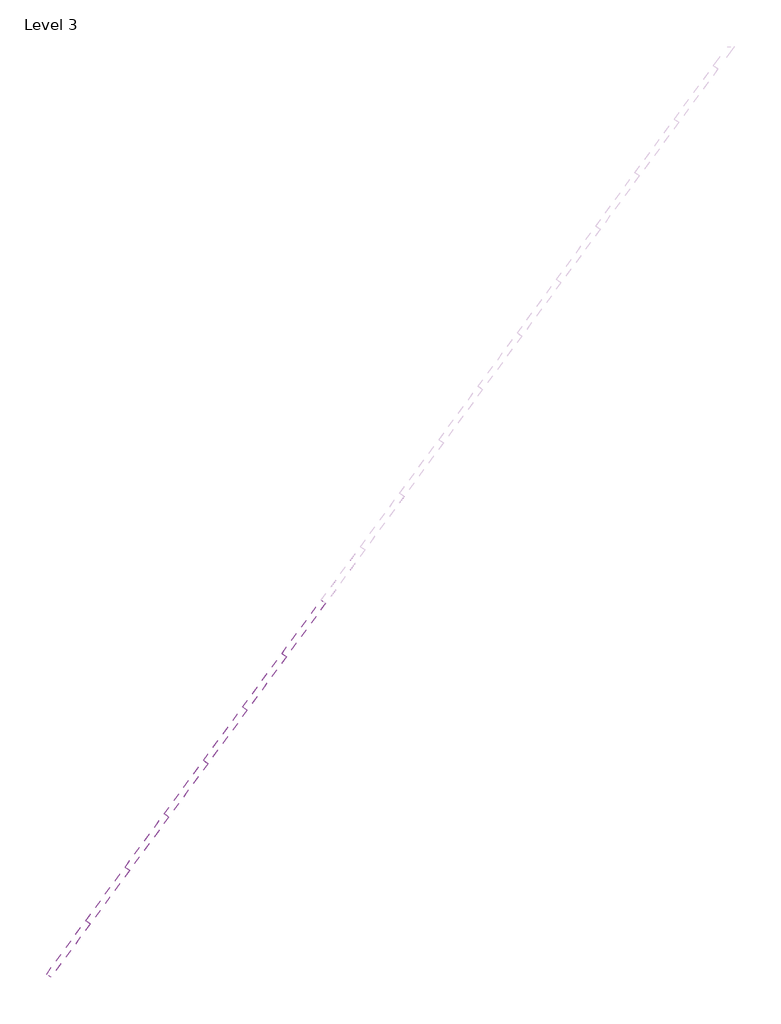
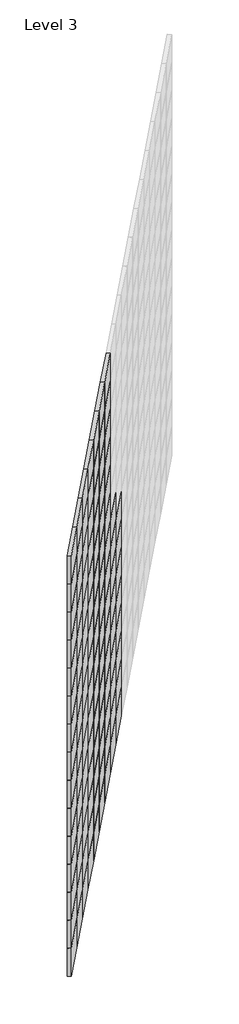
# One storey, part 1 of 9: 122 plates.
"""IFC4 building model written with IfcOpenShell, lengths in millimetres."""

import ifcopenshell
import ifcopenshell.guid

model = None  # the IFC model being written
_history = None  # IfcOwnerHistory: only IFC2X3 demands one
_inside = {}  # id of a spatial element -> (the spatial element, [elements in it])
_under = {}  # id of a project, library or spatial element -> (it, [spatial elements below it])
_declared = {}  # id of a project -> (the project, [libraries it declares])
_typed = {}  # id of a type object -> (the type object, [elements of that type])
_made_of = {}  # id of a material, layer set ... -> (it, [elements and type objects made of it])


def new_model(schema):
    """Start an empty IFC model of exactly this schema.

    Asked for "IFC4X3", IfcOpenShell would pick the latest addendum, in which some entities
    have other attributes; the version numbers below select the first issue.
    IFC2X3 requires an IfcOwnerHistory on every rooted entity: one is made here for all.
    """
    global model, _history
    if schema == "IFC4X3":
        model = ifcopenshell.file(schema_version=(4, 3, 0, 0))
    else:
        model = ifcopenshell.file(schema=schema)
    _inside.clear()
    _under.clear()
    _declared.clear()
    _typed.clear()
    _made_of.clear()
    _history = None
    if model.schema == "IFC2X3":
        org = make("IfcOrganization", Name="unknown")
        user = make(
            "IfcPersonAndOrganization",
            ThePerson=make("IfcPerson", FamilyName="unknown"),
            TheOrganization=org,
        )
        app = make(
            "IfcApplication",
            ApplicationDeveloper=org,
            Version="unknown",
            ApplicationFullName="unknown",
            ApplicationIdentifier="unknown",
        )
        _history = make(
            "IfcOwnerHistory",
            OwningUser=user,
            OwningApplication=app,
            ChangeAction="ADDED",
            CreationDate=0,
        )
    return model


def make(cls, **values):
    """One entity of the class cls with the attributes given. An attribute that is None is left unset."""
    return model.create_entity(
        cls, **{name: value for name, value in values.items() if value is not None}
    )


def rooted(cls, **values):
    """An entity with a GlobalId (a new one), such as an element, a storey or a relation."""
    return make(cls, GlobalId=ifcopenshell.guid.new(), OwnerHistory=_history, **values)


def si_unit(unit_type, name, prefix=None):
    """IfcSIUnit, for example si_unit("LENGTHUNIT", "METRE", prefix="MILLI")."""
    return make("IfcSIUnit", UnitType=unit_type, Prefix=prefix, Name=name)


def assignment(units):
    """IfcUnitAssignment: the units of a project."""
    return None if units is None else make("IfcUnitAssignment", Units=units)


def point(xyz):
    """IfcCartesianPoint."""
    return None if xyz is None else make("IfcCartesianPoint", Coordinates=xyz)


def direction(xyz):
    """IfcDirection."""
    return None if xyz is None else make("IfcDirection", DirectionRatios=xyz)


def frame(location, z_axis=None, x_axis=None):
    """IfcAxis2Placement3D, a coordinate frame: its origin and axes. An axis left out is left unset."""
    return make(
        "IfcAxis2Placement3D",
        Location=point(location),
        Axis=direction(z_axis),
        RefDirection=direction(x_axis),
    )


def origin():
    """The frame at (0, 0, 0) with its axes left unset."""
    return frame((0.0, 0.0, 0.0))


def origin_with_axes():
    """The frame at (0, 0, 0) with the z axis (0, 0, 1) and the x axis (1, 0, 0) written out."""
    return frame((0.0, 0.0, 0.0), z_axis=(0.0, 0.0, 1.0), x_axis=(1.0, 0.0, 0.0))


def place(relative_to, where):
    """IfcLocalPlacement: puts the frame where relative to a parent placement (None: the world)."""
    return make(
        "IfcLocalPlacement", PlacementRelTo=relative_to, RelativePlacement=where
    )


def context(
    kind, dimensions, precision=None, world=None, true_north=None, identifier=None
):
    """IfcGeometricRepresentationContext, for example the 3D "Model" context."""
    return make(
        "IfcGeometricRepresentationContext",
        ContextIdentifier=identifier,
        ContextType=kind,
        CoordinateSpaceDimension=dimensions,
        Precision=precision,
        WorldCoordinateSystem=world,
        TrueNorth=true_north,
    )


def project(units=None, contexts=None):
    """IfcProject with its units and contexts."""
    return rooted(
        "IfcProject",
        Name="project",
        RepresentationContexts=contexts,
        UnitsInContext=assignment(units),
    )


def spatial(cls, under=None, at=None, **own):
    """A site, building, storey or space (cls), placed at a placement, below another one or the project."""
    s = rooted(cls, ObjectPlacement=at, **own)
    if under is not None:
        _under.setdefault(under.id(), (under, []))[1].append(s)
    return s


def polyline(points):
    """IfcPolyline through the points."""
    return make("IfcPolyline", Points=[point(p) for p in points])


def outline(outer, holes=None, kind="AREA"):
    """IfcArbitraryClosedProfileDef: a profile drawn as a closed curve; with holes, ...WithVoids."""
    if holes is None:
        return make("IfcArbitraryClosedProfileDef", ProfileType=kind, OuterCurve=outer)
    return make(
        "IfcArbitraryProfileDefWithVoids",
        ProfileType=kind,
        OuterCurve=outer,
        InnerCurves=holes,
    )


def extrude(swept, where, along, depth):
    """IfcExtrudedAreaSolid: the profile swept, set in the frame where, extruded along a direction by depth."""
    return make(
        "IfcExtrudedAreaSolid",
        SweptArea=swept,
        Position=where,
        ExtrudedDirection=direction(along),
        Depth=depth,
    )


def shape(context_of_items, identifier, shape_type, items):
    """IfcShapeRepresentation: the items that make up one representation, for example the "Body"."""
    return make(
        "IfcShapeRepresentation",
        ContextOfItems=context_of_items,
        RepresentationIdentifier=identifier,
        RepresentationType=shape_type,
        Items=items,
    )


def source(mapping_origin, context_of_items, identifier, shape_type, items):
    """IfcRepresentationMap: a shape defined once, which mapped items show again and again."""
    return make(
        "IfcRepresentationMap",
        MappingOrigin=mapping_origin,
        MappedRepresentation=shape(context_of_items, identifier, shape_type, items),
    )


def transform(
    local_origin,
    x_axis=None,
    y_axis=None,
    z_axis=None,
    scale=None,
    scale2=None,
    scale3=None,
    uniform=True,
):
    """IfcCartesianTransformationOperator3D, or its non-uniform kind. x_axis, y_axis, z_axis: its Axis1, 2, 3."""
    if uniform:
        return make(
            "IfcCartesianTransformationOperator3D",
            Axis1=direction(x_axis),
            Axis2=direction(y_axis),
            LocalOrigin=point(local_origin),
            Scale=scale,
            Axis3=direction(z_axis),
        )
    return make(
        "IfcCartesianTransformationOperator3DnonUniform",
        Axis1=direction(x_axis),
        Axis2=direction(y_axis),
        LocalOrigin=point(local_origin),
        Scale=scale,
        Axis3=direction(z_axis),
        Scale2=scale2,
        Scale3=scale3,
    )


def mapped(mapping_source, mapping_target):
    """IfcMappedItem: shows the shape of a source again, moved by a transform."""
    return make(
        "IfcMappedItem", MappingSource=mapping_source, MappingTarget=mapping_target
    )


def made_of(thing, what):
    """Note that an element or type object is made of a material, layer set ...; save() writes the relation."""
    if what is not None:
        _made_of.setdefault(what.id(), (what, []))[1].append(thing)
    return thing


def element(
    cls,
    number,
    at=None,
    inside=None,
    cuts=None,
    type_object=None,
    material=None,
    context=None,
    identifier="Body",
    shape_type=None,
    held_by="IfcProductDefinitionShape",
    body=None,
    shapes=None,
    **own,
):
    """One element of the class cls, such as IfcWall. Its Tag is "e" and its number.

    at: its placement. inside: the storey or other place that contains it. cuts: it is an
    opening in that element (IfcRelVoidsElement). A single representation is given by context,
    identifier, shape_type and body (its items); several are given by shapes. held_by: the class
    of the entity that holds the representations. save() writes the other relations.
    """
    e = rooted(cls, Tag="e%d" % number, ObjectPlacement=at, **own)
    if body is not None:
        shapes = [shape(context, identifier, shape_type, body)]
    if shapes is not None:
        e.Representation = make(held_by, Representations=shapes)
    if inside is not None:
        _inside.setdefault(inside.id(), (inside, []))[1].append(e)
    if cuts is not None:
        rooted(
            "IfcRelVoidsElement", RelatingBuildingElement=cuts, RelatedOpeningElement=e
        )
    if type_object is not None:
        _typed.setdefault(type_object.id(), (type_object, []))[1].append(e)
    return made_of(e, material)


def aggregate(whole, parts):
    """IfcRelAggregates: a whole, such as a stair, and the parts it consists of."""
    return rooted("IfcRelAggregates", RelatingObject=whole, RelatedObjects=parts)


def save(model, path):
    """Write the relations noted so far, then the file.

    IfcRelAggregates (storeys below a building ...), IfcRelContainedInSpatialStructure (elements
    in a storey), IfcRelDefinesByType, IfcRelAssociatesMaterial and IfcRelDeclares: one each for
    every whole, place, type object, material and project.
    """
    for whole, parts in _under.values():
        aggregate(whole, parts)
    for where, things in _inside.values():
        rooted(
            "IfcRelContainedInSpatialStructure",
            RelatedElements=things,
            RelatingStructure=where,
        )
    for kind, things in _typed.values():
        rooted("IfcRelDefinesByType", RelatedObjects=things, RelatingType=kind)
    for what, things in _made_of.values():
        rooted("IfcRelAssociatesMaterial", RelatedObjects=things, RelatingMaterial=what)
    for by, libraries in _declared.values():
        rooted("IfcRelDeclares", RelatingContext=by, RelatedDefinitions=libraries)
    model.write(path)


def system_panel_glazed_2fc8f5ca(model_context):
    return source(origin(), model_context, "Body", "SweptSolid", [
        extrude(outline(polyline([(148.4832393, 24.5), (-148.4832393, 24.5), (-148.4832393, 49.5), (148.4832393, 49.5), (148.4832393, 24.5)])), origin_with_axes(), (0.0, 0.0, 1.0), 200.0),
    ])


model = new_model("IFC4")

# Units and contexts
model_context = context("Model", 3, world=origin())
ifc_project = project(units=[si_unit("LENGTHUNIT", "METRE", prefix="MILLI")], contexts=[model_context])

# Site, building, storey
site = spatial("IfcSite", under=ifc_project)
building = spatial("IfcBuilding", under=site)
storey = spatial("IfcBuildingStorey", under=building, Name="Level 3", Elevation=22950.0)

# Plates
placement = place(None, origin())
system_panel_glazed_shape = system_panel_glazed_2fc8f5ca(model_context)
element("IfcPlate", 1, ObjectType="System Panel : Glazed", at=placement, inside=storey, context=model_context, shape_type="MappedRepresentation", body=[
    mapped(system_panel_glazed_shape, transform((-37416.3631886, 22522.5700791, 35100.0), x_axis=(0.5920548138930122, 0.8058976965757569, 0.0), y_axis=(-0.8058976965757569, 0.5920548138930122, 0.0), z_axis=(0.0, 0.0, 1.0))),
])
element("IfcPlate", 2, ObjectType="System Panel : Glazed", at=placement, inside=storey, context=model_context, shape_type="MappedRepresentation", body=[
    mapped(system_panel_glazed_shape, transform((-37240.5427555, 22761.8946801, 35100.0), x_axis=(0.5920548138930122, 0.8058976965757569, 0.0), y_axis=(-0.8058976965757569, 0.5920548138930122, 0.0), z_axis=(0.0, 0.0, 1.0))),
])
element("IfcPlate", 3, ObjectType="System Panel : Glazed", at=placement, inside=storey, context=model_context, shape_type="MappedRepresentation", body=[
    mapped(system_panel_glazed_shape, transform((-37064.7223224, 23001.2192809, 35100.0), x_axis=(0.5920548138930122, 0.8058976965757569, 0.0), y_axis=(-0.8058976965757569, 0.5920548138930122, 0.0), z_axis=(0.0, 0.0, 1.0))),
])
element("IfcPlate", 4, ObjectType="System Panel : Glazed", at=placement, inside=storey, context=model_context, shape_type="MappedRepresentation", body=[
    mapped(system_panel_glazed_shape, transform((-36888.9018893, 23240.5438818, 35100.0), x_axis=(0.5920548138930122, 0.8058976965757569, 0.0), y_axis=(-0.8058976965757569, 0.5920548138930122, 0.0), z_axis=(0.0, 0.0, 1.0))),
])
element("IfcPlate", 5, ObjectType="System Panel : Glazed", at=placement, inside=storey, context=model_context, shape_type="MappedRepresentation", body=[
    mapped(system_panel_glazed_shape, transform((-36713.0814563, 23479.8684826, 35100.0), x_axis=(0.5920548138930122, 0.8058976965757569, 0.0), y_axis=(-0.8058976965757569, 0.5920548138930122, 0.0), z_axis=(0.0, 0.0, 1.0))),
])
element("IfcPlate", 6, ObjectType="System Panel : Glazed", at=placement, inside=storey, context=model_context, shape_type="MappedRepresentation", body=[
    mapped(system_panel_glazed_shape, transform((-36537.2610232, 23719.1930834, 35100.0), x_axis=(0.5920548138930122, 0.8058976965757569, 0.0), y_axis=(-0.8058976965757569, 0.5920548138930122, 0.0), z_axis=(0.0, 0.0, 1.0))),
])
element("IfcPlate", 7, ObjectType="System Panel : Glazed", at=placement, inside=storey, context=model_context, shape_type="MappedRepresentation", body=[
    mapped(system_panel_glazed_shape, transform((-36361.4405902, 23958.5176843, 35100.0), x_axis=(0.5920548138930122, 0.8058976965757569, 0.0), y_axis=(-0.8058976965757569, 0.5920548138930122, 0.0), z_axis=(0.0, 0.0, 1.0))),
])
element("IfcPlate", 8, ObjectType="System Panel : Glazed", at=placement, inside=storey, context=model_context, shape_type="MappedRepresentation", body=[
    mapped(system_panel_glazed_shape, transform((-36185.6201571, 24197.8422851, 35100.0), x_axis=(0.5920548138930122, 0.8058976965757569, 0.0), y_axis=(-0.8058976965757569, 0.5920548138930122, 0.0), z_axis=(0.0, 0.0, 1.0))),
])
element("IfcPlate", 9, ObjectType="System Panel : Glazed", at=placement, inside=storey, context=model_context, shape_type="MappedRepresentation", body=[
    mapped(system_panel_glazed_shape, transform((-36009.7997241, 24437.166886, 35100.0), x_axis=(0.5920548138930122, 0.8058976965757569, 0.0), y_axis=(-0.8058976965757569, 0.5920548138930122, 0.0), z_axis=(0.0, 0.0, 1.0))),
])
element("IfcPlate", 10, ObjectType="System Panel : Glazed", at=placement, inside=storey, context=model_context, shape_type="MappedRepresentation", body=[
    mapped(system_panel_glazed_shape, transform((-37416.3631886, 22522.5700791, 35300.0), x_axis=(0.5920548138930122, 0.8058976965757569, 0.0), y_axis=(-0.8058976965757569, 0.5920548138930122, 0.0), z_axis=(0.0, 0.0, 1.0))),
])
element("IfcPlate", 11, ObjectType="System Panel : Glazed", at=placement, inside=storey, context=model_context, shape_type="MappedRepresentation", body=[
    mapped(system_panel_glazed_shape, transform((-37240.5427555, 22761.8946801, 35300.0), x_axis=(0.5920548138930122, 0.8058976965757569, 0.0), y_axis=(-0.8058976965757569, 0.5920548138930122, 0.0), z_axis=(0.0, 0.0, 1.0))),
])
element("IfcPlate", 12, ObjectType="System Panel : Glazed", at=placement, inside=storey, context=model_context, shape_type="MappedRepresentation", body=[
    mapped(system_panel_glazed_shape, transform((-37064.7223224, 23001.2192809, 35300.0), x_axis=(0.5920548138930122, 0.8058976965757569, 0.0), y_axis=(-0.8058976965757569, 0.5920548138930122, 0.0), z_axis=(0.0, 0.0, 1.0))),
])
element("IfcPlate", 13, ObjectType="System Panel : Glazed", at=placement, inside=storey, context=model_context, shape_type="MappedRepresentation", body=[
    mapped(system_panel_glazed_shape, transform((-36888.9018893, 23240.5438818, 35300.0), x_axis=(0.5920548138930122, 0.8058976965757569, 0.0), y_axis=(-0.8058976965757569, 0.5920548138930122, 0.0), z_axis=(0.0, 0.0, 1.0))),
])
element("IfcPlate", 14, ObjectType="System Panel : Glazed", at=placement, inside=storey, context=model_context, shape_type="MappedRepresentation", body=[
    mapped(system_panel_glazed_shape, transform((-36713.0814563, 23479.8684826, 35300.0), x_axis=(0.5920548138930122, 0.8058976965757569, 0.0), y_axis=(-0.8058976965757569, 0.5920548138930122, 0.0), z_axis=(0.0, 0.0, 1.0))),
])
element("IfcPlate", 15, ObjectType="System Panel : Glazed", at=placement, inside=storey, context=model_context, shape_type="MappedRepresentation", body=[
    mapped(system_panel_glazed_shape, transform((-36537.2610232, 23719.1930834, 35300.0), x_axis=(0.5920548138930122, 0.8058976965757569, 0.0), y_axis=(-0.8058976965757569, 0.5920548138930122, 0.0), z_axis=(0.0, 0.0, 1.0))),
])
element("IfcPlate", 16, ObjectType="System Panel : Glazed", at=placement, inside=storey, context=model_context, shape_type="MappedRepresentation", body=[
    mapped(system_panel_glazed_shape, transform((-36361.4405902, 23958.5176843, 35300.0), x_axis=(0.5920548138930122, 0.8058976965757569, 0.0), y_axis=(-0.8058976965757569, 0.5920548138930122, 0.0), z_axis=(0.0, 0.0, 1.0))),
])
element("IfcPlate", 17, ObjectType="System Panel : Glazed", at=placement, inside=storey, context=model_context, shape_type="MappedRepresentation", body=[
    mapped(system_panel_glazed_shape, transform((-36185.6201571, 24197.8422851, 35300.0), x_axis=(0.5920548138930122, 0.8058976965757569, 0.0), y_axis=(-0.8058976965757569, 0.5920548138930122, 0.0), z_axis=(0.0, 0.0, 1.0))),
])
element("IfcPlate", 18, ObjectType="System Panel : Glazed", at=placement, inside=storey, context=model_context, shape_type="MappedRepresentation", body=[
    mapped(system_panel_glazed_shape, transform((-36009.7997241, 24437.166886, 35300.0), x_axis=(0.5920548138930122, 0.8058976965757569, 0.0), y_axis=(-0.8058976965757569, 0.5920548138930122, 0.0), z_axis=(0.0, 0.0, 1.0))),
])
element("IfcPlate", 19, ObjectType="System Panel : Glazed", at=placement, inside=storey, context=model_context, shape_type="MappedRepresentation", body=[
    mapped(system_panel_glazed_shape, transform((-37416.3631886, 22522.5700791, 35500.0), x_axis=(0.5920548138930122, 0.8058976965757569, 0.0), y_axis=(-0.8058976965757569, 0.5920548138930122, 0.0), z_axis=(0.0, 0.0, 1.0))),
])
element("IfcPlate", 20, ObjectType="System Panel : Glazed", at=placement, inside=storey, context=model_context, shape_type="MappedRepresentation", body=[
    mapped(system_panel_glazed_shape, transform((-37240.5427555, 22761.8946801, 35500.0), x_axis=(0.5920548138930122, 0.8058976965757569, 0.0), y_axis=(-0.8058976965757569, 0.5920548138930122, 0.0), z_axis=(0.0, 0.0, 1.0))),
])
element("IfcPlate", 21, ObjectType="System Panel : Glazed", at=placement, inside=storey, context=model_context, shape_type="MappedRepresentation", body=[
    mapped(system_panel_glazed_shape, transform((-37064.7223224, 23001.2192809, 35500.0), x_axis=(0.5920548138930122, 0.8058976965757569, 0.0), y_axis=(-0.8058976965757569, 0.5920548138930122, 0.0), z_axis=(0.0, 0.0, 1.0))),
])
element("IfcPlate", 22, ObjectType="System Panel : Glazed", at=placement, inside=storey, context=model_context, shape_type="MappedRepresentation", body=[
    mapped(system_panel_glazed_shape, transform((-36888.9018893, 23240.5438818, 35500.0), x_axis=(0.5920548138930122, 0.8058976965757569, 0.0), y_axis=(-0.8058976965757569, 0.5920548138930122, 0.0), z_axis=(0.0, 0.0, 1.0))),
])
element("IfcPlate", 23, ObjectType="System Panel : Glazed", at=placement, inside=storey, context=model_context, shape_type="MappedRepresentation", body=[
    mapped(system_panel_glazed_shape, transform((-36713.0814563, 23479.8684826, 35500.0), x_axis=(0.5920548138930122, 0.8058976965757569, 0.0), y_axis=(-0.8058976965757569, 0.5920548138930122, 0.0), z_axis=(0.0, 0.0, 1.0))),
])
element("IfcPlate", 24, ObjectType="System Panel : Glazed", at=placement, inside=storey, context=model_context, shape_type="MappedRepresentation", body=[
    mapped(system_panel_glazed_shape, transform((-36537.2610232, 23719.1930834, 35500.0), x_axis=(0.5920548138930122, 0.8058976965757569, 0.0), y_axis=(-0.8058976965757569, 0.5920548138930122, 0.0), z_axis=(0.0, 0.0, 1.0))),
])
element("IfcPlate", 25, ObjectType="System Panel : Glazed", at=placement, inside=storey, context=model_context, shape_type="MappedRepresentation", body=[
    mapped(system_panel_glazed_shape, transform((-36361.4405902, 23958.5176843, 35500.0), x_axis=(0.5920548138930122, 0.8058976965757569, 0.0), y_axis=(-0.8058976965757569, 0.5920548138930122, 0.0), z_axis=(0.0, 0.0, 1.0))),
])
element("IfcPlate", 26, ObjectType="System Panel : Glazed", at=placement, inside=storey, context=model_context, shape_type="MappedRepresentation", body=[
    mapped(system_panel_glazed_shape, transform((-36185.6201571, 24197.8422851, 35500.0), x_axis=(0.5920548138930122, 0.8058976965757569, 0.0), y_axis=(-0.8058976965757569, 0.5920548138930122, 0.0), z_axis=(0.0, 0.0, 1.0))),
])
element("IfcPlate", 27, ObjectType="System Panel : Glazed", at=placement, inside=storey, context=model_context, shape_type="MappedRepresentation", body=[
    mapped(system_panel_glazed_shape, transform((-36009.7997241, 24437.166886, 35500.0), x_axis=(0.5920548138930122, 0.8058976965757569, 0.0), y_axis=(-0.8058976965757569, 0.5920548138930122, 0.0), z_axis=(0.0, 0.0, 1.0))),
])
element("IfcPlate", 28, ObjectType="System Panel : Glazed", at=placement, inside=storey, context=model_context, shape_type="MappedRepresentation", body=[
    mapped(system_panel_glazed_shape, transform((-37416.3631886, 22522.5700791, 35700.0), x_axis=(0.5920548138930122, 0.8058976965757569, 0.0), y_axis=(-0.8058976965757569, 0.5920548138930122, 0.0), z_axis=(0.0, 0.0, 1.0))),
])
element("IfcPlate", 29, ObjectType="System Panel : Glazed", at=placement, inside=storey, context=model_context, shape_type="MappedRepresentation", body=[
    mapped(system_panel_glazed_shape, transform((-37240.5427555, 22761.8946801, 35700.0), x_axis=(0.5920548138930122, 0.8058976965757569, 0.0), y_axis=(-0.8058976965757569, 0.5920548138930122, 0.0), z_axis=(0.0, 0.0, 1.0))),
])
element("IfcPlate", 30, ObjectType="System Panel : Glazed", at=placement, inside=storey, context=model_context, shape_type="MappedRepresentation", body=[
    mapped(system_panel_glazed_shape, transform((-37064.7223224, 23001.2192809, 35700.0), x_axis=(0.5920548138930122, 0.8058976965757569, 0.0), y_axis=(-0.8058976965757569, 0.5920548138930122, 0.0), z_axis=(0.0, 0.0, 1.0))),
])
element("IfcPlate", 31, ObjectType="System Panel : Glazed", at=placement, inside=storey, context=model_context, shape_type="MappedRepresentation", body=[
    mapped(system_panel_glazed_shape, transform((-36888.9018893, 23240.5438818, 35700.0), x_axis=(0.5920548138930122, 0.8058976965757569, 0.0), y_axis=(-0.8058976965757569, 0.5920548138930122, 0.0), z_axis=(0.0, 0.0, 1.0))),
])
element("IfcPlate", 32, ObjectType="System Panel : Glazed", at=placement, inside=storey, context=model_context, shape_type="MappedRepresentation", body=[
    mapped(system_panel_glazed_shape, transform((-36713.0814563, 23479.8684826, 35700.0), x_axis=(0.5920548138930122, 0.8058976965757569, 0.0), y_axis=(-0.8058976965757569, 0.5920548138930122, 0.0), z_axis=(0.0, 0.0, 1.0))),
])
element("IfcPlate", 33, ObjectType="System Panel : Glazed", at=placement, inside=storey, context=model_context, shape_type="MappedRepresentation", body=[
    mapped(system_panel_glazed_shape, transform((-36537.2610232, 23719.1930834, 35700.0), x_axis=(0.5920548138930122, 0.8058976965757569, 0.0), y_axis=(-0.8058976965757569, 0.5920548138930122, 0.0), z_axis=(0.0, 0.0, 1.0))),
])
element("IfcPlate", 34, ObjectType="System Panel : Glazed", at=placement, inside=storey, context=model_context, shape_type="MappedRepresentation", body=[
    mapped(system_panel_glazed_shape, transform((-36361.4405902, 23958.5176843, 35700.0), x_axis=(0.5920548138930122, 0.8058976965757569, 0.0), y_axis=(-0.8058976965757569, 0.5920548138930122, 0.0), z_axis=(0.0, 0.0, 1.0))),
])
element("IfcPlate", 35, ObjectType="System Panel : Glazed", at=placement, inside=storey, context=model_context, shape_type="MappedRepresentation", body=[
    mapped(system_panel_glazed_shape, transform((-36185.6201571, 24197.8422851, 35700.0), x_axis=(0.5920548138930122, 0.8058976965757569, 0.0), y_axis=(-0.8058976965757569, 0.5920548138930122, 0.0), z_axis=(0.0, 0.0, 1.0))),
])
element("IfcPlate", 36, ObjectType="System Panel : Glazed", at=placement, inside=storey, context=model_context, shape_type="MappedRepresentation", body=[
    mapped(system_panel_glazed_shape, transform((-36009.7997241, 24437.166886, 35700.0), x_axis=(0.5920548138930122, 0.8058976965757569, 0.0), y_axis=(-0.8058976965757569, 0.5920548138930122, 0.0), z_axis=(0.0, 0.0, 1.0))),
])
element("IfcPlate", 37, ObjectType="System Panel : Glazed", at=placement, inside=storey, context=model_context, shape_type="MappedRepresentation", body=[
    mapped(system_panel_glazed_shape, transform((-37416.3631886, 22522.5700791, 35900.0), x_axis=(0.5920548138930122, 0.8058976965757569, 0.0), y_axis=(-0.8058976965757569, 0.5920548138930122, 0.0), z_axis=(0.0, 0.0, 1.0))),
])
element("IfcPlate", 38, ObjectType="System Panel : Glazed", at=placement, inside=storey, context=model_context, shape_type="MappedRepresentation", body=[
    mapped(system_panel_glazed_shape, transform((-37240.5427555, 22761.8946801, 35900.0), x_axis=(0.5920548138930122, 0.8058976965757569, 0.0), y_axis=(-0.8058976965757569, 0.5920548138930122, 0.0), z_axis=(0.0, 0.0, 1.0))),
])
element("IfcPlate", 39, ObjectType="System Panel : Glazed", at=placement, inside=storey, context=model_context, shape_type="MappedRepresentation", body=[
    mapped(system_panel_glazed_shape, transform((-37064.7223224, 23001.2192809, 35900.0), x_axis=(0.5920548138930122, 0.8058976965757569, 0.0), y_axis=(-0.8058976965757569, 0.5920548138930122, 0.0), z_axis=(0.0, 0.0, 1.0))),
])
element("IfcPlate", 40, ObjectType="System Panel : Glazed", at=placement, inside=storey, context=model_context, shape_type="MappedRepresentation", body=[
    mapped(system_panel_glazed_shape, transform((-36888.9018893, 23240.5438818, 35900.0), x_axis=(0.5920548138930122, 0.8058976965757569, 0.0), y_axis=(-0.8058976965757569, 0.5920548138930122, 0.0), z_axis=(0.0, 0.0, 1.0))),
])
element("IfcPlate", 41, ObjectType="System Panel : Glazed", at=placement, inside=storey, context=model_context, shape_type="MappedRepresentation", body=[
    mapped(system_panel_glazed_shape, transform((-36713.0814563, 23479.8684826, 35900.0), x_axis=(0.5920548138930122, 0.8058976965757569, 0.0), y_axis=(-0.8058976965757569, 0.5920548138930122, 0.0), z_axis=(0.0, 0.0, 1.0))),
])
element("IfcPlate", 42, ObjectType="System Panel : Glazed", at=placement, inside=storey, context=model_context, shape_type="MappedRepresentation", body=[
    mapped(system_panel_glazed_shape, transform((-36537.2610232, 23719.1930834, 35900.0), x_axis=(0.5920548138930122, 0.8058976965757569, 0.0), y_axis=(-0.8058976965757569, 0.5920548138930122, 0.0), z_axis=(0.0, 0.0, 1.0))),
])
element("IfcPlate", 43, ObjectType="System Panel : Glazed", at=placement, inside=storey, context=model_context, shape_type="MappedRepresentation", body=[
    mapped(system_panel_glazed_shape, transform((-36361.4405902, 23958.5176843, 35900.0), x_axis=(0.5920548138930122, 0.8058976965757569, 0.0), y_axis=(-0.8058976965757569, 0.5920548138930122, 0.0), z_axis=(0.0, 0.0, 1.0))),
])
element("IfcPlate", 44, ObjectType="System Panel : Glazed", at=placement, inside=storey, context=model_context, shape_type="MappedRepresentation", body=[
    mapped(system_panel_glazed_shape, transform((-36185.6201571, 24197.8422851, 35900.0), x_axis=(0.5920548138930122, 0.8058976965757569, 0.0), y_axis=(-0.8058976965757569, 0.5920548138930122, 0.0), z_axis=(0.0, 0.0, 1.0))),
])
element("IfcPlate", 45, ObjectType="System Panel : Glazed", at=placement, inside=storey, context=model_context, shape_type="MappedRepresentation", body=[
    mapped(system_panel_glazed_shape, transform((-36009.7997241, 24437.166886, 35900.0), x_axis=(0.5920548138930122, 0.8058976965757569, 0.0), y_axis=(-0.8058976965757569, 0.5920548138930122, 0.0), z_axis=(0.0, 0.0, 1.0))),
])
element("IfcPlate", 46, ObjectType="System Panel : Glazed", at=placement, inside=storey, context=model_context, shape_type="MappedRepresentation", body=[
    mapped(system_panel_glazed_shape, transform((-37416.3631886, 22522.5700791, 36100.0), x_axis=(0.5920548138930122, 0.8058976965757569, 0.0), y_axis=(-0.8058976965757569, 0.5920548138930122, 0.0), z_axis=(0.0, 0.0, 1.0))),
])
element("IfcPlate", 47, ObjectType="System Panel : Glazed", at=placement, inside=storey, context=model_context, shape_type="MappedRepresentation", body=[
    mapped(system_panel_glazed_shape, transform((-37240.5427555, 22761.8946801, 36100.0), x_axis=(0.5920548138930122, 0.8058976965757569, 0.0), y_axis=(-0.8058976965757569, 0.5920548138930122, 0.0), z_axis=(0.0, 0.0, 1.0))),
])
element("IfcPlate", 48, ObjectType="System Panel : Glazed", at=placement, inside=storey, context=model_context, shape_type="MappedRepresentation", body=[
    mapped(system_panel_glazed_shape, transform((-37064.7223224, 23001.2192809, 36100.0), x_axis=(0.5920548138930122, 0.8058976965757569, 0.0), y_axis=(-0.8058976965757569, 0.5920548138930122, 0.0), z_axis=(0.0, 0.0, 1.0))),
])
element("IfcPlate", 49, ObjectType="System Panel : Glazed", at=placement, inside=storey, context=model_context, shape_type="MappedRepresentation", body=[
    mapped(system_panel_glazed_shape, transform((-36888.9018893, 23240.5438818, 36100.0), x_axis=(0.5920548138930122, 0.8058976965757569, 0.0), y_axis=(-0.8058976965757569, 0.5920548138930122, 0.0), z_axis=(0.0, 0.0, 1.0))),
])
element("IfcPlate", 50, ObjectType="System Panel : Glazed", at=placement, inside=storey, context=model_context, shape_type="MappedRepresentation", body=[
    mapped(system_panel_glazed_shape, transform((-36713.0814563, 23479.8684826, 36100.0), x_axis=(0.5920548138930122, 0.8058976965757569, 0.0), y_axis=(-0.8058976965757569, 0.5920548138930122, 0.0), z_axis=(0.0, 0.0, 1.0))),
])
element("IfcPlate", 51, ObjectType="System Panel : Glazed", at=placement, inside=storey, context=model_context, shape_type="MappedRepresentation", body=[
    mapped(system_panel_glazed_shape, transform((-36537.2610232, 23719.1930834, 36100.0), x_axis=(0.5920548138930122, 0.8058976965757569, 0.0), y_axis=(-0.8058976965757569, 0.5920548138930122, 0.0), z_axis=(0.0, 0.0, 1.0))),
])
element("IfcPlate", 52, ObjectType="System Panel : Glazed", at=placement, inside=storey, context=model_context, shape_type="MappedRepresentation", body=[
    mapped(system_panel_glazed_shape, transform((-36361.4405902, 23958.5176843, 36100.0), x_axis=(0.5920548138930122, 0.8058976965757569, 0.0), y_axis=(-0.8058976965757569, 0.5920548138930122, 0.0), z_axis=(0.0, 0.0, 1.0))),
])
element("IfcPlate", 53, ObjectType="System Panel : Glazed", at=placement, inside=storey, context=model_context, shape_type="MappedRepresentation", body=[
    mapped(system_panel_glazed_shape, transform((-36185.6201571, 24197.8422851, 36100.0), x_axis=(0.5920548138930122, 0.8058976965757569, 0.0), y_axis=(-0.8058976965757569, 0.5920548138930122, 0.0), z_axis=(0.0, 0.0, 1.0))),
])
element("IfcPlate", 54, ObjectType="System Panel : Glazed", at=placement, inside=storey, context=model_context, shape_type="MappedRepresentation", body=[
    mapped(system_panel_glazed_shape, transform((-36009.7997241, 24437.166886, 36100.0), x_axis=(0.5920548138930122, 0.8058976965757569, 0.0), y_axis=(-0.8058976965757569, 0.5920548138930122, 0.0), z_axis=(0.0, 0.0, 1.0))),
])
element("IfcPlate", 55, ObjectType="System Panel : Glazed", at=placement, inside=storey, context=model_context, shape_type="MappedRepresentation", body=[
    mapped(system_panel_glazed_shape, transform((-37416.3631886, 22522.5700791, 36300.0), x_axis=(0.5920548138930122, 0.8058976965757569, 0.0), y_axis=(-0.8058976965757569, 0.5920548138930122, 0.0), z_axis=(0.0, 0.0, 1.0))),
])
element("IfcPlate", 56, ObjectType="System Panel : Glazed", at=placement, inside=storey, context=model_context, shape_type="MappedRepresentation", body=[
    mapped(system_panel_glazed_shape, transform((-37240.5427555, 22761.8946801, 36300.0), x_axis=(0.5920548138930122, 0.8058976965757569, 0.0), y_axis=(-0.8058976965757569, 0.5920548138930122, 0.0), z_axis=(0.0, 0.0, 1.0))),
])
element("IfcPlate", 57, ObjectType="System Panel : Glazed", at=placement, inside=storey, context=model_context, shape_type="MappedRepresentation", body=[
    mapped(system_panel_glazed_shape, transform((-37064.7223224, 23001.2192809, 36300.0), x_axis=(0.5920548138930122, 0.8058976965757569, 0.0), y_axis=(-0.8058976965757569, 0.5920548138930122, 0.0), z_axis=(0.0, 0.0, 1.0))),
])
element("IfcPlate", 58, ObjectType="System Panel : Glazed", at=placement, inside=storey, context=model_context, shape_type="MappedRepresentation", body=[
    mapped(system_panel_glazed_shape, transform((-36888.9018893, 23240.5438818, 36300.0), x_axis=(0.5920548138930122, 0.8058976965757569, 0.0), y_axis=(-0.8058976965757569, 0.5920548138930122, 0.0), z_axis=(0.0, 0.0, 1.0))),
])
element("IfcPlate", 59, ObjectType="System Panel : Glazed", at=placement, inside=storey, context=model_context, shape_type="MappedRepresentation", body=[
    mapped(system_panel_glazed_shape, transform((-36713.0814563, 23479.8684826, 36300.0), x_axis=(0.5920548138930122, 0.8058976965757569, 0.0), y_axis=(-0.8058976965757569, 0.5920548138930122, 0.0), z_axis=(0.0, 0.0, 1.0))),
])
element("IfcPlate", 60, ObjectType="System Panel : Glazed", at=placement, inside=storey, context=model_context, shape_type="MappedRepresentation", body=[
    mapped(system_panel_glazed_shape, transform((-36537.2610232, 23719.1930834, 36300.0), x_axis=(0.5920548138930122, 0.8058976965757569, 0.0), y_axis=(-0.8058976965757569, 0.5920548138930122, 0.0), z_axis=(0.0, 0.0, 1.0))),
])
element("IfcPlate", 61, ObjectType="System Panel : Glazed", at=placement, inside=storey, context=model_context, shape_type="MappedRepresentation", body=[
    mapped(system_panel_glazed_shape, transform((-36361.4405902, 23958.5176843, 36300.0), x_axis=(0.5920548138930122, 0.8058976965757569, 0.0), y_axis=(-0.8058976965757569, 0.5920548138930122, 0.0), z_axis=(0.0, 0.0, 1.0))),
])
element("IfcPlate", 62, ObjectType="System Panel : Glazed", at=placement, inside=storey, context=model_context, shape_type="MappedRepresentation", body=[
    mapped(system_panel_glazed_shape, transform((-36185.6201571, 24197.8422851, 36300.0), x_axis=(0.5920548138930122, 0.8058976965757569, 0.0), y_axis=(-0.8058976965757569, 0.5920548138930122, 0.0), z_axis=(0.0, 0.0, 1.0))),
])
element("IfcPlate", 63, ObjectType="System Panel : Glazed", at=placement, inside=storey, context=model_context, shape_type="MappedRepresentation", body=[
    mapped(system_panel_glazed_shape, transform((-36009.7997241, 24437.166886, 36300.0), x_axis=(0.5920548138930122, 0.8058976965757569, 0.0), y_axis=(-0.8058976965757569, 0.5920548138930122, 0.0), z_axis=(0.0, 0.0, 1.0))),
])
element("IfcPlate", 64, ObjectType="System Panel : Glazed", at=placement, inside=storey, context=model_context, shape_type="MappedRepresentation", body=[
    mapped(system_panel_glazed_shape, transform((-37416.3631886, 22522.5700791, 36500.0), x_axis=(0.5920548138930122, 0.8058976965757569, 0.0), y_axis=(-0.8058976965757569, 0.5920548138930122, 0.0), z_axis=(0.0, 0.0, 1.0))),
])
element("IfcPlate", 65, ObjectType="System Panel : Glazed", at=placement, inside=storey, context=model_context, shape_type="MappedRepresentation", body=[
    mapped(system_panel_glazed_shape, transform((-37240.5427555, 22761.8946801, 36500.0), x_axis=(0.5920548138930122, 0.8058976965757569, 0.0), y_axis=(-0.8058976965757569, 0.5920548138930122, 0.0), z_axis=(0.0, 0.0, 1.0))),
])
element("IfcPlate", 66, ObjectType="System Panel : Glazed", at=placement, inside=storey, context=model_context, shape_type="MappedRepresentation", body=[
    mapped(system_panel_glazed_shape, transform((-37064.7223224, 23001.2192809, 36500.0), x_axis=(0.5920548138930122, 0.8058976965757569, 0.0), y_axis=(-0.8058976965757569, 0.5920548138930122, 0.0), z_axis=(0.0, 0.0, 1.0))),
])
element("IfcPlate", 67, ObjectType="System Panel : Glazed", at=placement, inside=storey, context=model_context, shape_type="MappedRepresentation", body=[
    mapped(system_panel_glazed_shape, transform((-36888.9018893, 23240.5438818, 36500.0), x_axis=(0.5920548138930122, 0.8058976965757569, 0.0), y_axis=(-0.8058976965757569, 0.5920548138930122, 0.0), z_axis=(0.0, 0.0, 1.0))),
])
element("IfcPlate", 68, ObjectType="System Panel : Glazed", at=placement, inside=storey, context=model_context, shape_type="MappedRepresentation", body=[
    mapped(system_panel_glazed_shape, transform((-36713.0814563, 23479.8684826, 36500.0), x_axis=(0.5920548138930122, 0.8058976965757569, 0.0), y_axis=(-0.8058976965757569, 0.5920548138930122, 0.0), z_axis=(0.0, 0.0, 1.0))),
])
element("IfcPlate", 69, ObjectType="System Panel : Glazed", at=placement, inside=storey, context=model_context, shape_type="MappedRepresentation", body=[
    mapped(system_panel_glazed_shape, transform((-36537.2610232, 23719.1930834, 36500.0), x_axis=(0.5920548138930122, 0.8058976965757569, 0.0), y_axis=(-0.8058976965757569, 0.5920548138930122, 0.0), z_axis=(0.0, 0.0, 1.0))),
])
element("IfcPlate", 70, ObjectType="System Panel : Glazed", at=placement, inside=storey, context=model_context, shape_type="MappedRepresentation", body=[
    mapped(system_panel_glazed_shape, transform((-36361.4405902, 23958.5176843, 36500.0), x_axis=(0.5920548138930122, 0.8058976965757569, 0.0), y_axis=(-0.8058976965757569, 0.5920548138930122, 0.0), z_axis=(0.0, 0.0, 1.0))),
])
element("IfcPlate", 71, ObjectType="System Panel : Glazed", at=placement, inside=storey, context=model_context, shape_type="MappedRepresentation", body=[
    mapped(system_panel_glazed_shape, transform((-36185.6201571, 24197.8422851, 36500.0), x_axis=(0.5920548138930122, 0.8058976965757569, 0.0), y_axis=(-0.8058976965757569, 0.5920548138930122, 0.0), z_axis=(0.0, 0.0, 1.0))),
])
element("IfcPlate", 72, ObjectType="System Panel : Glazed", at=placement, inside=storey, context=model_context, shape_type="MappedRepresentation", body=[
    mapped(system_panel_glazed_shape, transform((-36009.7997241, 24437.166886, 36500.0), x_axis=(0.5920548138930122, 0.8058976965757569, 0.0), y_axis=(-0.8058976965757569, 0.5920548138930122, 0.0), z_axis=(0.0, 0.0, 1.0))),
])
element("IfcPlate", 73, ObjectType="System Panel : Glazed", at=placement, inside=storey, context=model_context, shape_type="MappedRepresentation", body=[
    mapped(system_panel_glazed_shape, transform((-37416.3631886, 22522.5700791, 36700.0), x_axis=(0.5920548138930122, 0.8058976965757569, 0.0), y_axis=(-0.8058976965757569, 0.5920548138930122, 0.0), z_axis=(0.0, 0.0, 1.0))),
])
element("IfcPlate", 74, ObjectType="System Panel : Glazed", at=placement, inside=storey, context=model_context, shape_type="MappedRepresentation", body=[
    mapped(system_panel_glazed_shape, transform((-37240.5427555, 22761.8946801, 36700.0), x_axis=(0.5920548138930122, 0.8058976965757569, 0.0), y_axis=(-0.8058976965757569, 0.5920548138930122, 0.0), z_axis=(0.0, 0.0, 1.0))),
])
element("IfcPlate", 75, ObjectType="System Panel : Glazed", at=placement, inside=storey, context=model_context, shape_type="MappedRepresentation", body=[
    mapped(system_panel_glazed_shape, transform((-37064.7223224, 23001.2192809, 36700.0), x_axis=(0.5920548138930122, 0.8058976965757569, 0.0), y_axis=(-0.8058976965757569, 0.5920548138930122, 0.0), z_axis=(0.0, 0.0, 1.0))),
])
element("IfcPlate", 76, ObjectType="System Panel : Glazed", at=placement, inside=storey, context=model_context, shape_type="MappedRepresentation", body=[
    mapped(system_panel_glazed_shape, transform((-36888.9018893, 23240.5438818, 36700.0), x_axis=(0.5920548138930122, 0.8058976965757569, 0.0), y_axis=(-0.8058976965757569, 0.5920548138930122, 0.0), z_axis=(0.0, 0.0, 1.0))),
])
element("IfcPlate", 77, ObjectType="System Panel : Glazed", at=placement, inside=storey, context=model_context, shape_type="MappedRepresentation", body=[
    mapped(system_panel_glazed_shape, transform((-36713.0814563, 23479.8684826, 36700.0), x_axis=(0.5920548138930122, 0.8058976965757569, 0.0), y_axis=(-0.8058976965757569, 0.5920548138930122, 0.0), z_axis=(0.0, 0.0, 1.0))),
])
element("IfcPlate", 78, ObjectType="System Panel : Glazed", at=placement, inside=storey, context=model_context, shape_type="MappedRepresentation", body=[
    mapped(system_panel_glazed_shape, transform((-36537.2610232, 23719.1930834, 36700.0), x_axis=(0.5920548138930122, 0.8058976965757569, 0.0), y_axis=(-0.8058976965757569, 0.5920548138930122, 0.0), z_axis=(0.0, 0.0, 1.0))),
])
element("IfcPlate", 79, ObjectType="System Panel : Glazed", at=placement, inside=storey, context=model_context, shape_type="MappedRepresentation", body=[
    mapped(system_panel_glazed_shape, transform((-36361.4405902, 23958.5176843, 36700.0), x_axis=(0.5920548138930122, 0.8058976965757569, 0.0), y_axis=(-0.8058976965757569, 0.5920548138930122, 0.0), z_axis=(0.0, 0.0, 1.0))),
])
element("IfcPlate", 80, ObjectType="System Panel : Glazed", at=placement, inside=storey, context=model_context, shape_type="MappedRepresentation", body=[
    mapped(system_panel_glazed_shape, transform((-36185.6201571, 24197.8422851, 36700.0), x_axis=(0.5920548138930122, 0.8058976965757569, 0.0), y_axis=(-0.8058976965757569, 0.5920548138930122, 0.0), z_axis=(0.0, 0.0, 1.0))),
])
element("IfcPlate", 81, ObjectType="System Panel : Glazed", at=placement, inside=storey, context=model_context, shape_type="MappedRepresentation", body=[
    mapped(system_panel_glazed_shape, transform((-37416.3631886, 22522.5700791, 36900.0), x_axis=(0.5920548138930122, 0.8058976965757569, 0.0), y_axis=(-0.8058976965757569, 0.5920548138930122, 0.0), z_axis=(0.0, 0.0, 1.0))),
])
element("IfcPlate", 82, ObjectType="System Panel : Glazed", at=placement, inside=storey, context=model_context, shape_type="MappedRepresentation", body=[
    mapped(system_panel_glazed_shape, transform((-37240.5427555, 22761.8946801, 36900.0), x_axis=(0.5920548138930122, 0.8058976965757569, 0.0), y_axis=(-0.8058976965757569, 0.5920548138930122, 0.0), z_axis=(0.0, 0.0, 1.0))),
])
element("IfcPlate", 83, ObjectType="System Panel : Glazed", at=placement, inside=storey, context=model_context, shape_type="MappedRepresentation", body=[
    mapped(system_panel_glazed_shape, transform((-37064.7223224, 23001.2192809, 36900.0), x_axis=(0.5920548138930122, 0.8058976965757569, 0.0), y_axis=(-0.8058976965757569, 0.5920548138930122, 0.0), z_axis=(0.0, 0.0, 1.0))),
])
element("IfcPlate", 84, ObjectType="System Panel : Glazed", at=placement, inside=storey, context=model_context, shape_type="MappedRepresentation", body=[
    mapped(system_panel_glazed_shape, transform((-36888.9018893, 23240.5438818, 36900.0), x_axis=(0.5920548138930122, 0.8058976965757569, 0.0), y_axis=(-0.8058976965757569, 0.5920548138930122, 0.0), z_axis=(0.0, 0.0, 1.0))),
])
element("IfcPlate", 85, ObjectType="System Panel : Glazed", at=placement, inside=storey, context=model_context, shape_type="MappedRepresentation", body=[
    mapped(system_panel_glazed_shape, transform((-36713.0814563, 23479.8684826, 36900.0), x_axis=(0.5920548138930122, 0.8058976965757569, 0.0), y_axis=(-0.8058976965757569, 0.5920548138930122, 0.0), z_axis=(0.0, 0.0, 1.0))),
])
element("IfcPlate", 86, ObjectType="System Panel : Glazed", at=placement, inside=storey, context=model_context, shape_type="MappedRepresentation", body=[
    mapped(system_panel_glazed_shape, transform((-36537.2610232, 23719.1930834, 36900.0), x_axis=(0.5920548138930122, 0.8058976965757569, 0.0), y_axis=(-0.8058976965757569, 0.5920548138930122, 0.0), z_axis=(0.0, 0.0, 1.0))),
])
element("IfcPlate", 87, ObjectType="System Panel : Glazed", at=placement, inside=storey, context=model_context, shape_type="MappedRepresentation", body=[
    mapped(system_panel_glazed_shape, transform((-36361.4405902, 23958.5176843, 36900.0), x_axis=(0.5920548138930122, 0.8058976965757569, 0.0), y_axis=(-0.8058976965757569, 0.5920548138930122, 0.0), z_axis=(0.0, 0.0, 1.0))),
])
element("IfcPlate", 88, ObjectType="System Panel : Glazed", at=placement, inside=storey, context=model_context, shape_type="MappedRepresentation", body=[
    mapped(system_panel_glazed_shape, transform((-37416.3631886, 22522.5700791, 37100.0), x_axis=(0.5920548138930122, 0.8058976965757569, 0.0), y_axis=(-0.8058976965757569, 0.5920548138930122, 0.0), z_axis=(0.0, 0.0, 1.0))),
])
element("IfcPlate", 89, ObjectType="System Panel : Glazed", at=placement, inside=storey, context=model_context, shape_type="MappedRepresentation", body=[
    mapped(system_panel_glazed_shape, transform((-37240.5427555, 22761.8946801, 37100.0), x_axis=(0.5920548138930122, 0.8058976965757569, 0.0), y_axis=(-0.8058976965757569, 0.5920548138930122, 0.0), z_axis=(0.0, 0.0, 1.0))),
])
element("IfcPlate", 90, ObjectType="System Panel : Glazed", at=placement, inside=storey, context=model_context, shape_type="MappedRepresentation", body=[
    mapped(system_panel_glazed_shape, transform((-37064.7223224, 23001.2192809, 37100.0), x_axis=(0.5920548138930122, 0.8058976965757569, 0.0), y_axis=(-0.8058976965757569, 0.5920548138930122, 0.0), z_axis=(0.0, 0.0, 1.0))),
])
element("IfcPlate", 91, ObjectType="System Panel : Glazed", at=placement, inside=storey, context=model_context, shape_type="MappedRepresentation", body=[
    mapped(system_panel_glazed_shape, transform((-36888.9018893, 23240.5438818, 37100.0), x_axis=(0.5920548138930122, 0.8058976965757569, 0.0), y_axis=(-0.8058976965757569, 0.5920548138930122, 0.0), z_axis=(0.0, 0.0, 1.0))),
])
element("IfcPlate", 92, ObjectType="System Panel : Glazed", at=placement, inside=storey, context=model_context, shape_type="MappedRepresentation", body=[
    mapped(system_panel_glazed_shape, transform((-36713.0814563, 23479.8684826, 37100.0), x_axis=(0.5920548138930122, 0.8058976965757569, 0.0), y_axis=(-0.8058976965757569, 0.5920548138930122, 0.0), z_axis=(0.0, 0.0, 1.0))),
])
element("IfcPlate", 93, ObjectType="System Panel : Glazed", at=placement, inside=storey, context=model_context, shape_type="MappedRepresentation", body=[
    mapped(system_panel_glazed_shape, transform((-36537.2610232, 23719.1930834, 37100.0), x_axis=(0.5920548138930122, 0.8058976965757569, 0.0), y_axis=(-0.8058976965757569, 0.5920548138930122, 0.0), z_axis=(0.0, 0.0, 1.0))),
])
element("IfcPlate", 94, ObjectType="System Panel : Glazed", at=placement, inside=storey, context=model_context, shape_type="MappedRepresentation", body=[
    mapped(system_panel_glazed_shape, transform((-36361.4405902, 23958.5176843, 37100.0), x_axis=(0.5920548138930122, 0.8058976965757569, 0.0), y_axis=(-0.8058976965757569, 0.5920548138930122, 0.0), z_axis=(0.0, 0.0, 1.0))),
])
element("IfcPlate", 95, ObjectType="System Panel : Glazed", at=placement, inside=storey, context=model_context, shape_type="MappedRepresentation", body=[
    mapped(system_panel_glazed_shape, transform((-37416.3631886, 22522.5700791, 37300.0), x_axis=(0.5920548138930122, 0.8058976965757569, 0.0), y_axis=(-0.8058976965757569, 0.5920548138930122, 0.0), z_axis=(0.0, 0.0, 1.0))),
])
element("IfcPlate", 96, ObjectType="System Panel : Glazed", at=placement, inside=storey, context=model_context, shape_type="MappedRepresentation", body=[
    mapped(system_panel_glazed_shape, transform((-37240.5427555, 22761.8946801, 37300.0), x_axis=(0.5920548138930122, 0.8058976965757569, 0.0), y_axis=(-0.8058976965757569, 0.5920548138930122, 0.0), z_axis=(0.0, 0.0, 1.0))),
])
element("IfcPlate", 97, ObjectType="System Panel : Glazed", at=placement, inside=storey, context=model_context, shape_type="MappedRepresentation", body=[
    mapped(system_panel_glazed_shape, transform((-37064.7223224, 23001.2192809, 37300.0), x_axis=(0.5920548138930122, 0.8058976965757569, 0.0), y_axis=(-0.8058976965757569, 0.5920548138930122, 0.0), z_axis=(0.0, 0.0, 1.0))),
])
element("IfcPlate", 98, ObjectType="System Panel : Glazed", at=placement, inside=storey, context=model_context, shape_type="MappedRepresentation", body=[
    mapped(system_panel_glazed_shape, transform((-36888.9018893, 23240.5438818, 37300.0), x_axis=(0.5920548138930122, 0.8058976965757569, 0.0), y_axis=(-0.8058976965757569, 0.5920548138930122, 0.0), z_axis=(0.0, 0.0, 1.0))),
])
element("IfcPlate", 99, ObjectType="System Panel : Glazed", at=placement, inside=storey, context=model_context, shape_type="MappedRepresentation", body=[
    mapped(system_panel_glazed_shape, transform((-36713.0814563, 23479.8684826, 37300.0), x_axis=(0.5920548138930122, 0.8058976965757569, 0.0), y_axis=(-0.8058976965757569, 0.5920548138930122, 0.0), z_axis=(0.0, 0.0, 1.0))),
])
element("IfcPlate", 100, ObjectType="System Panel : Glazed", at=placement, inside=storey, context=model_context, shape_type="MappedRepresentation", body=[
    mapped(system_panel_glazed_shape, transform((-36537.2610232, 23719.1930834, 37300.0), x_axis=(0.5920548138930122, 0.8058976965757569, 0.0), y_axis=(-0.8058976965757569, 0.5920548138930122, 0.0), z_axis=(0.0, 0.0, 1.0))),
])
element("IfcPlate", 101, ObjectType="System Panel : Glazed", at=placement, inside=storey, context=model_context, shape_type="MappedRepresentation", body=[
    mapped(system_panel_glazed_shape, transform((-36361.4405902, 23958.5176843, 37300.0), x_axis=(0.5920548138930122, 0.8058976965757569, 0.0), y_axis=(-0.8058976965757569, 0.5920548138930122, 0.0), z_axis=(0.0, 0.0, 1.0))),
])
element("IfcPlate", 102, ObjectType="System Panel : Glazed", at=placement, inside=storey, context=model_context, shape_type="MappedRepresentation", body=[
    mapped(system_panel_glazed_shape, transform((-37416.3631886, 22522.5700791, 37500.0), x_axis=(0.5920548138930122, 0.8058976965757569, 0.0), y_axis=(-0.8058976965757569, 0.5920548138930122, 0.0), z_axis=(0.0, 0.0, 1.0))),
])
element("IfcPlate", 103, ObjectType="System Panel : Glazed", at=placement, inside=storey, context=model_context, shape_type="MappedRepresentation", body=[
    mapped(system_panel_glazed_shape, transform((-37240.5427555, 22761.8946801, 37500.0), x_axis=(0.5920548138930122, 0.8058976965757569, 0.0), y_axis=(-0.8058976965757569, 0.5920548138930122, 0.0), z_axis=(0.0, 0.0, 1.0))),
])
element("IfcPlate", 104, ObjectType="System Panel : Glazed", at=placement, inside=storey, context=model_context, shape_type="MappedRepresentation", body=[
    mapped(system_panel_glazed_shape, transform((-37064.7223224, 23001.2192809, 37500.0), x_axis=(0.5920548138930122, 0.8058976965757569, 0.0), y_axis=(-0.8058976965757569, 0.5920548138930122, 0.0), z_axis=(0.0, 0.0, 1.0))),
])
element("IfcPlate", 105, ObjectType="System Panel : Glazed", at=placement, inside=storey, context=model_context, shape_type="MappedRepresentation", body=[
    mapped(system_panel_glazed_shape, transform((-36888.9018893, 23240.5438818, 37500.0), x_axis=(0.5920548138930122, 0.8058976965757569, 0.0), y_axis=(-0.8058976965757569, 0.5920548138930122, 0.0), z_axis=(0.0, 0.0, 1.0))),
])
element("IfcPlate", 106, ObjectType="System Panel : Glazed", at=placement, inside=storey, context=model_context, shape_type="MappedRepresentation", body=[
    mapped(system_panel_glazed_shape, transform((-36713.0814563, 23479.8684826, 37500.0), x_axis=(0.5920548138930122, 0.8058976965757569, 0.0), y_axis=(-0.8058976965757569, 0.5920548138930122, 0.0), z_axis=(0.0, 0.0, 1.0))),
])
element("IfcPlate", 107, ObjectType="System Panel : Glazed", at=placement, inside=storey, context=model_context, shape_type="MappedRepresentation", body=[
    mapped(system_panel_glazed_shape, transform((-36537.2610232, 23719.1930834, 37500.0), x_axis=(0.5920548138930122, 0.8058976965757569, 0.0), y_axis=(-0.8058976965757569, 0.5920548138930122, 0.0), z_axis=(0.0, 0.0, 1.0))),
])
element("IfcPlate", 108, ObjectType="System Panel : Glazed", at=placement, inside=storey, context=model_context, shape_type="MappedRepresentation", body=[
    mapped(system_panel_glazed_shape, transform((-36361.4405902, 23958.5176843, 37500.0), x_axis=(0.5920548138930122, 0.8058976965757569, 0.0), y_axis=(-0.8058976965757569, 0.5920548138930122, 0.0), z_axis=(0.0, 0.0, 1.0))),
])
element("IfcPlate", 109, ObjectType="System Panel : Glazed", at=placement, inside=storey, context=model_context, shape_type="MappedRepresentation", body=[
    mapped(system_panel_glazed_shape, transform((-37416.3631886, 22522.5700791, 37700.0), x_axis=(0.5920548138930122, 0.8058976965757569, 0.0), y_axis=(-0.8058976965757569, 0.5920548138930122, 0.0), z_axis=(0.0, 0.0, 1.0))),
])
element("IfcPlate", 110, ObjectType="System Panel : Glazed", at=placement, inside=storey, context=model_context, shape_type="MappedRepresentation", body=[
    mapped(system_panel_glazed_shape, transform((-37240.5427555, 22761.8946801, 37700.0), x_axis=(0.5920548138930122, 0.8058976965757569, 0.0), y_axis=(-0.8058976965757569, 0.5920548138930122, 0.0), z_axis=(0.0, 0.0, 1.0))),
])
element("IfcPlate", 111, ObjectType="System Panel : Glazed", at=placement, inside=storey, context=model_context, shape_type="MappedRepresentation", body=[
    mapped(system_panel_glazed_shape, transform((-37064.7223224, 23001.2192809, 37700.0), x_axis=(0.5920548138930122, 0.8058976965757569, 0.0), y_axis=(-0.8058976965757569, 0.5920548138930122, 0.0), z_axis=(0.0, 0.0, 1.0))),
])
element("IfcPlate", 112, ObjectType="System Panel : Glazed", at=placement, inside=storey, context=model_context, shape_type="MappedRepresentation", body=[
    mapped(system_panel_glazed_shape, transform((-36888.9018893, 23240.5438818, 37700.0), x_axis=(0.5920548138930122, 0.8058976965757569, 0.0), y_axis=(-0.8058976965757569, 0.5920548138930122, 0.0), z_axis=(0.0, 0.0, 1.0))),
])
element("IfcPlate", 113, ObjectType="System Panel : Glazed", at=placement, inside=storey, context=model_context, shape_type="MappedRepresentation", body=[
    mapped(system_panel_glazed_shape, transform((-36713.0814563, 23479.8684826, 37700.0), x_axis=(0.5920548138930122, 0.8058976965757569, 0.0), y_axis=(-0.8058976965757569, 0.5920548138930122, 0.0), z_axis=(0.0, 0.0, 1.0))),
])
element("IfcPlate", 114, ObjectType="System Panel : Glazed", at=placement, inside=storey, context=model_context, shape_type="MappedRepresentation", body=[
    mapped(system_panel_glazed_shape, transform((-36537.2610232, 23719.1930834, 37700.0), x_axis=(0.5920548138930122, 0.8058976965757569, 0.0), y_axis=(-0.8058976965757569, 0.5920548138930122, 0.0), z_axis=(0.0, 0.0, 1.0))),
])
element("IfcPlate", 115, ObjectType="System Panel : Glazed", at=placement, inside=storey, context=model_context, shape_type="MappedRepresentation", body=[
    mapped(system_panel_glazed_shape, transform((-36361.4405902, 23958.5176843, 37700.0), x_axis=(0.5920548138930122, 0.8058976965757569, 0.0), y_axis=(-0.8058976965757569, 0.5920548138930122, 0.0), z_axis=(0.0, 0.0, 1.0))),
])
element("IfcPlate", 116, ObjectType="System Panel : Glazed", at=placement, inside=storey, context=model_context, shape_type="MappedRepresentation", body=[
    mapped(system_panel_glazed_shape, transform((-37416.3631886, 22522.5700791, 37900.0), x_axis=(0.5920548138930122, 0.8058976965757569, 0.0), y_axis=(-0.8058976965757569, 0.5920548138930122, 0.0), z_axis=(0.0, 0.0, 1.0))),
])
element("IfcPlate", 117, ObjectType="System Panel : Glazed", at=placement, inside=storey, context=model_context, shape_type="MappedRepresentation", body=[
    mapped(system_panel_glazed_shape, transform((-37240.5427555, 22761.8946801, 37900.0), x_axis=(0.5920548138930122, 0.8058976965757569, 0.0), y_axis=(-0.8058976965757569, 0.5920548138930122, 0.0), z_axis=(0.0, 0.0, 1.0))),
])
element("IfcPlate", 118, ObjectType="System Panel : Glazed", at=placement, inside=storey, context=model_context, shape_type="MappedRepresentation", body=[
    mapped(system_panel_glazed_shape, transform((-37064.7223224, 23001.2192809, 37900.0), x_axis=(0.5920548138930122, 0.8058976965757569, 0.0), y_axis=(-0.8058976965757569, 0.5920548138930122, 0.0), z_axis=(0.0, 0.0, 1.0))),
])
element("IfcPlate", 119, ObjectType="System Panel : Glazed", at=placement, inside=storey, context=model_context, shape_type="MappedRepresentation", body=[
    mapped(system_panel_glazed_shape, transform((-36888.9018893, 23240.5438818, 37900.0), x_axis=(0.5920548138930122, 0.8058976965757569, 0.0), y_axis=(-0.8058976965757569, 0.5920548138930122, 0.0), z_axis=(0.0, 0.0, 1.0))),
])
element("IfcPlate", 120, ObjectType="System Panel : Glazed", at=placement, inside=storey, context=model_context, shape_type="MappedRepresentation", body=[
    mapped(system_panel_glazed_shape, transform((-36713.0814563, 23479.8684826, 37900.0), x_axis=(0.5920548138930122, 0.8058976965757569, 0.0), y_axis=(-0.8058976965757569, 0.5920548138930122, 0.0), z_axis=(0.0, 0.0, 1.0))),
])
element("IfcPlate", 121, ObjectType="System Panel : Glazed", at=placement, inside=storey, context=model_context, shape_type="MappedRepresentation", body=[
    mapped(system_panel_glazed_shape, transform((-36537.2610232, 23719.1930834, 37900.0), x_axis=(0.5920548138930122, 0.8058976965757569, 0.0), y_axis=(-0.8058976965757569, 0.5920548138930122, 0.0), z_axis=(0.0, 0.0, 1.0))),
])
element("IfcPlate", 122, ObjectType="System Panel : Glazed", at=placement, inside=storey, context=model_context, shape_type="MappedRepresentation", body=[
    mapped(system_panel_glazed_shape, transform((-36361.4405902, 23958.5176843, 37900.0), x_axis=(0.5920548138930122, 0.8058976965757569, 0.0), y_axis=(-0.8058976965757569, 0.5920548138930122, 0.0), z_axis=(0.0, 0.0, 1.0))),
])

save(model, "model.ifc")

# Revit data of these elements
# Project information
#   Project Issue Date = "05/22/2020"
#   Project Status = "Project  Status"
#   Project Address = "## Street\nCity, State  Zip"
#   Project Number = "1"
# Elements 1, 2, 3, 4, 5, 6, 7, 8, 9, 10, 11, 12, 13, 14, 15, 16, 17, 18, 19, 20, 21, 22, 23, 24, 25, 26, 27, 28, 29, 30, 31, 32, 33, 34, 35, 36, 37, 38, 39, 40, 41, 42, 43, 44, 45, 46, 47, 48, 49, 50, 51, 52, 53, 54, 55, 56, 57, 58, 59, 60, 61, 62, 63, 64, 65, 66, 67, 68, 69, 70, 71, 72, 73, 74, 75, 76, 77, 78, 79, 80, 81, 82, 83, 84, 85, 86, 87, 88, 89, 90, 91, 92, 93, 94, 95, 96, 97, 98, 99, 100, 101, 102, 103, 104, 105, 106, 107, 108, 109, 110, 111, 112, 113, 114, 115, 116, 117, 118, 119, 120, 121, 122 (IfcPlate, "System Panel : Glazed")
#   Phase Created = New Construction
#   Materials on its faces: "Glass"
# Materials
#   "Glass": class "Glass", colour RGB 218 227 224, transparency 0.85, Description = "Soda Lime Glass", Cost = 0
